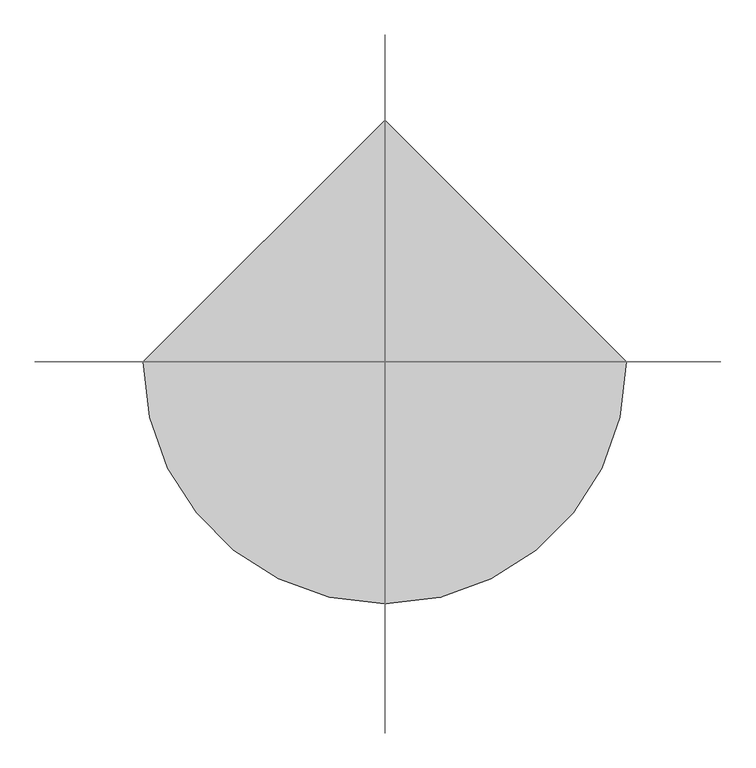
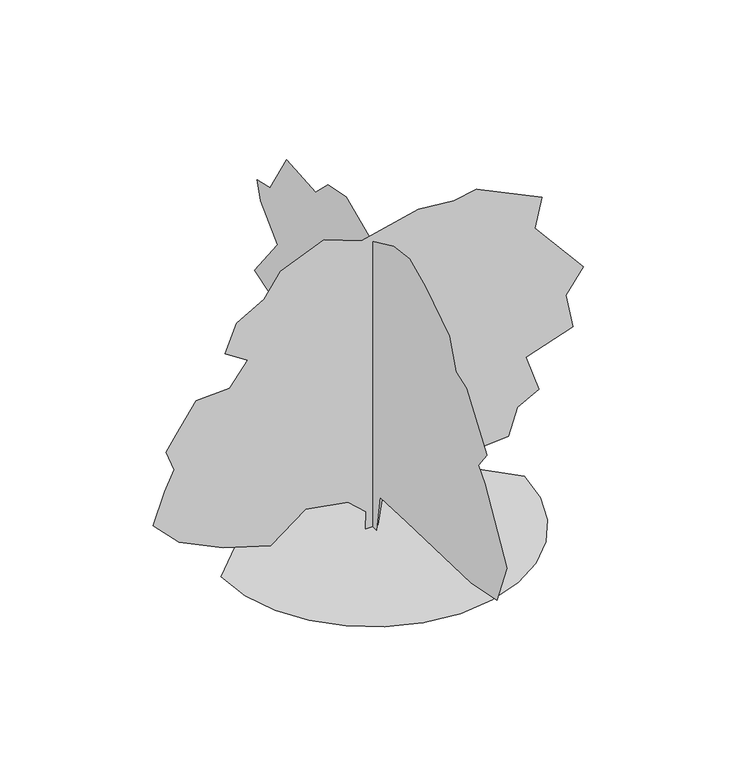
"""IFC4 building model written with IfcOpenShell, lengths in millimetres: proxy geometry, hibiscus syriacus 26076 : hibiscus syriacus 26076."""

import ifcopenshell
import ifcopenshell.guid

model = None  # the IFC model being written
_history = None  # IfcOwnerHistory: only IFC2X3 demands one
_inside = {}  # id of a spatial element -> (the spatial element, [elements in it])
_under = {}  # id of a project, library or spatial element -> (it, [spatial elements below it])
_declared = {}  # id of a project -> (the project, [libraries it declares])
_typed = {}  # id of a type object -> (the type object, [elements of that type])
_made_of = {}  # id of a material, layer set ... -> (it, [elements and type objects made of it])


def new_model(schema):
    """Start an empty IFC model of exactly this schema.

    Asked for "IFC4X3", IfcOpenShell would pick the latest addendum, in which some entities
    have other attributes; the version numbers below select the first issue.
    IFC2X3 requires an IfcOwnerHistory on every rooted entity: one is made here for all.
    """
    global model, _history
    if schema == "IFC4X3":
        model = ifcopenshell.file(schema_version=(4, 3, 0, 0))
    else:
        model = ifcopenshell.file(schema=schema)
    _inside.clear()
    _under.clear()
    _declared.clear()
    _typed.clear()
    _made_of.clear()
    _history = None
    if model.schema == "IFC2X3":
        org = make("IfcOrganization", Name="unknown")
        user = make(
            "IfcPersonAndOrganization",
            ThePerson=make("IfcPerson", FamilyName="unknown"),
            TheOrganization=org,
        )
        app = make(
            "IfcApplication",
            ApplicationDeveloper=org,
            Version="unknown",
            ApplicationFullName="unknown",
            ApplicationIdentifier="unknown",
        )
        _history = make(
            "IfcOwnerHistory",
            OwningUser=user,
            OwningApplication=app,
            ChangeAction="ADDED",
            CreationDate=0,
        )
    return model


def make(cls, **values):
    """One entity of the class cls with the attributes given. An attribute that is None is left unset."""
    return model.create_entity(
        cls, **{name: value for name, value in values.items() if value is not None}
    )


def rooted(cls, **values):
    """An entity with a GlobalId (a new one), such as an element, a storey or a relation."""
    return make(cls, GlobalId=ifcopenshell.guid.new(), OwnerHistory=_history, **values)


def si_unit(unit_type, name, prefix=None):
    """IfcSIUnit, for example si_unit("LENGTHUNIT", "METRE", prefix="MILLI")."""
    return make("IfcSIUnit", UnitType=unit_type, Prefix=prefix, Name=name)


def assignment(units):
    """IfcUnitAssignment: the units of a project."""
    return None if units is None else make("IfcUnitAssignment", Units=units)


def point(xyz):
    """IfcCartesianPoint."""
    return None if xyz is None else make("IfcCartesianPoint", Coordinates=xyz)


def direction(xyz):
    """IfcDirection."""
    return None if xyz is None else make("IfcDirection", DirectionRatios=xyz)


def frame(location, z_axis=None, x_axis=None):
    """IfcAxis2Placement3D, a coordinate frame: its origin and axes. An axis left out is left unset."""
    return make(
        "IfcAxis2Placement3D",
        Location=point(location),
        Axis=direction(z_axis),
        RefDirection=direction(x_axis),
    )


def origin():
    """The frame at (0, 0, 0) with its axes left unset."""
    return frame((0.0, 0.0, 0.0))


def place(relative_to, where):
    """IfcLocalPlacement: puts the frame where relative to a parent placement (None: the world)."""
    return make(
        "IfcLocalPlacement", PlacementRelTo=relative_to, RelativePlacement=where
    )


def context(
    kind, dimensions, precision=None, world=None, true_north=None, identifier=None
):
    """IfcGeometricRepresentationContext, for example the 3D "Model" context."""
    return make(
        "IfcGeometricRepresentationContext",
        ContextIdentifier=identifier,
        ContextType=kind,
        CoordinateSpaceDimension=dimensions,
        Precision=precision,
        WorldCoordinateSystem=world,
        TrueNorth=true_north,
    )


def project(units=None, contexts=None):
    """IfcProject with its units and contexts."""
    return rooted(
        "IfcProject",
        Name="project",
        RepresentationContexts=contexts,
        UnitsInContext=assignment(units),
    )


def spatial(cls, under=None, at=None, **own):
    """A site, building, storey or space (cls), placed at a placement, below another one or the project."""
    s = rooted(cls, ObjectPlacement=at, **own)
    if under is not None:
        _under.setdefault(under.id(), (under, []))[1].append(s)
    return s


def point_list(points):
    """IfcCartesianPointList2D or 3D."""
    cls = (
        "IfcCartesianPointList2D" if len(points[0]) == 2 else "IfcCartesianPointList3D"
    )
    return make(cls, CoordList=points)


def triangles(points, corners, closed=None, point_numbers=None):
    """IfcTriangulatedFaceSet: each triangle names its three corners, points numbered from 1."""
    return make(
        "IfcTriangulatedFaceSet",
        Coordinates=point_list(points),
        Closed=closed,
        CoordIndex=corners,
        PnIndex=point_numbers,
    )


def shape(context_of_items, identifier, shape_type, items):
    """IfcShapeRepresentation: the items that make up one representation, for example the "Body"."""
    return make(
        "IfcShapeRepresentation",
        ContextOfItems=context_of_items,
        RepresentationIdentifier=identifier,
        RepresentationType=shape_type,
        Items=items,
    )


def source(mapping_origin, context_of_items, identifier, shape_type, items):
    """IfcRepresentationMap: a shape defined once, which mapped items show again and again."""
    return make(
        "IfcRepresentationMap",
        MappingOrigin=mapping_origin,
        MappedRepresentation=shape(context_of_items, identifier, shape_type, items),
    )


def transform(
    local_origin,
    x_axis=None,
    y_axis=None,
    z_axis=None,
    scale=None,
    scale2=None,
    scale3=None,
    uniform=True,
):
    """IfcCartesianTransformationOperator3D, or its non-uniform kind. x_axis, y_axis, z_axis: its Axis1, 2, 3."""
    if uniform:
        return make(
            "IfcCartesianTransformationOperator3D",
            Axis1=direction(x_axis),
            Axis2=direction(y_axis),
            LocalOrigin=point(local_origin),
            Scale=scale,
            Axis3=direction(z_axis),
        )
    return make(
        "IfcCartesianTransformationOperator3DnonUniform",
        Axis1=direction(x_axis),
        Axis2=direction(y_axis),
        LocalOrigin=point(local_origin),
        Scale=scale,
        Axis3=direction(z_axis),
        Scale2=scale2,
        Scale3=scale3,
    )


def mapped(mapping_source, mapping_target):
    """IfcMappedItem: shows the shape of a source again, moved by a transform."""
    return make(
        "IfcMappedItem", MappingSource=mapping_source, MappingTarget=mapping_target
    )


def made_of(thing, what):
    """Note that an element or type object is made of a material, layer set ...; save() writes the relation."""
    if what is not None:
        _made_of.setdefault(what.id(), (what, []))[1].append(thing)
    return thing


def element(
    cls,
    number,
    at=None,
    inside=None,
    cuts=None,
    type_object=None,
    material=None,
    context=None,
    identifier="Body",
    shape_type=None,
    held_by="IfcProductDefinitionShape",
    body=None,
    shapes=None,
    **own,
):
    """One element of the class cls, such as IfcWall. Its Tag is "e" and its number.

    at: its placement. inside: the storey or other place that contains it. cuts: it is an
    opening in that element (IfcRelVoidsElement). A single representation is given by context,
    identifier, shape_type and body (its items); several are given by shapes. held_by: the class
    of the entity that holds the representations. save() writes the other relations.
    """
    e = rooted(cls, Tag="e%d" % number, ObjectPlacement=at, **own)
    if body is not None:
        shapes = [shape(context, identifier, shape_type, body)]
    if shapes is not None:
        e.Representation = make(held_by, Representations=shapes)
    if inside is not None:
        _inside.setdefault(inside.id(), (inside, []))[1].append(e)
    if cuts is not None:
        rooted(
            "IfcRelVoidsElement", RelatingBuildingElement=cuts, RelatedOpeningElement=e
        )
    if type_object is not None:
        _typed.setdefault(type_object.id(), (type_object, []))[1].append(e)
    return made_of(e, material)


def aggregate(whole, parts):
    """IfcRelAggregates: a whole, such as a stair, and the parts it consists of."""
    return rooted("IfcRelAggregates", RelatingObject=whole, RelatedObjects=parts)


def save(model, path):
    """Write the relations noted so far, then the file.

    IfcRelAggregates (storeys below a building ...), IfcRelContainedInSpatialStructure (elements
    in a storey), IfcRelDefinesByType, IfcRelAssociatesMaterial and IfcRelDeclares: one each for
    every whole, place, type object, material and project.
    """
    for whole, parts in _under.values():
        aggregate(whole, parts)
    for where, things in _inside.values():
        rooted(
            "IfcRelContainedInSpatialStructure",
            RelatedElements=things,
            RelatingStructure=where,
        )
    for kind, things in _typed.values():
        rooted("IfcRelDefinesByType", RelatedObjects=things, RelatingType=kind)
    for what, things in _made_of.values():
        rooted("IfcRelAssociatesMaterial", RelatedObjects=things, RelatingMaterial=what)
    for by, libraries in _declared.values():
        rooted("IfcRelDeclares", RelatingContext=by, RelatedDefinitions=libraries)
    model.write(path)


def entourage_edde2c96(model_context):
    return source(origin(), model_context, "Body", "Tessellation", [
        triangles([(-718.2296339, 0.0, 5.8e-05), (-699.2430748, -164.5709867, 5.8e-05), (-645.166361, -315.7023142, 5.8e-05), (-560.3301876, -449.0652858, 5.8e-05), (-449.0652858, -560.3301876, 5.8e-05), (-315.7023142, -645.166361, 5.8e-05), (-164.5707324, -699.2430748, 5.8e-05), (3.14e-05, -718.2296339, 5.8e-05), (164.5709867, -699.2430748, 5.8e-05), (315.7023142, -645.166361, 5.8e-05), (449.0652858, -560.3301876, 5.8e-05), (560.3301876, -449.0652858, 5.8e-05), (645.166361, -315.7023142, 5.8e-05), (699.2430748, -164.5707324, 5.8e-05), (718.2296339, 6.28e-05, 5.8e-05), (-9.42e-05, 718.2296339, 5.8e-05), (-34.4417068, 8.54e-05, 0.0004029), (-31.4201161, 7.54e-05, 85.3357887), (-116.0190539, 6.6e-05, 163.8917949), (-318.4505839, 6.17e-05, 200.1483391), (-484.6279043, 7.68e-05, 73.2501891), (-708.2093153, 6.85e-05, 142.7419322), (-916.6853256, 5.67e-05, 242.4475559), (-1040.5638834, 4.15e-05, 369.3446795), (-986.1773048, 2.35e-05, 520.4140194), (-940.856016, 1.24e-05, 614.076689), (-980.1346504, 1e-07, 716.8046482), (-931.7932697, -8.2e-06, 786.2967001), (-838.1305275, -2.47e-05, 925.2806585), (-677.9959705, -2.55e-05, 931.323313), (-593.398518, -3.84e-05, 1040.0939993), (-699.1465691, -4.67e-05, 1109.5859785), (-644.762534, -6.29e-05, 1245.5473743), (-514.8412491, -7.16e-05, 1318.0593727), (-436.2865236, -8.53e-05, 1432.8727135), (-230.8316043, -9.53e-05, 1517.4726368), (-52.5699789, -8.74e-05, 1451.0008221), (216.3332524, -9.5e-05, 1514.4501469), (385.5321362, -9.28e-05, 1496.3220383), (491.2801509, -9.53e-05, 1517.4726368), (802.4816133, -7.77e-05, 1369.4233887), (769.2456333, -6.04e-05, 1224.3967758), (998.8722422, -2.8e-05, 952.4739841), (914.2723188, -1.43e-05, 837.6606434), (947.5082262, 5.9e-06, 668.4632675), (726.946907, 1.49e-05, 592.9286339), (787.37614, 3.65e-05, 411.6459128), (684.6481808, 4.3e-05, 357.2593343), (642.3495272, 5.85e-05, 227.340611), (237.483106, 6.21e-05, 197.1267394), (140.7988277, 7.07e-05, 124.6136692), (53.1785627, 6.42e-05, 178.9984673), (25.9860297, 8.59e-05, 0.0), (-0.0007807, 31.0927106, 0.000457), (-0.0007807, 31.0927106, 100.9481805), (-0.0007869, 87.072138, 68.5389896), (-0.0007995, 193.1381747, 80.3241033), (-0.0008058, 269.7409118, 130.4109715), (-0.0008121, 346.3449205, 98.0017761), (-0.0008373, 520.1752622, 192.282958), (-0.0008373, 470.0888935, 354.3281542), (-0.0008562, 649.8120077, 383.7922351), (-0.0008688, 764.7167673, 489.857745), (-0.0008688, 747.0383406, 566.4617901), (-0.0008877, 891.4071447, 584.1376734), (-0.0008814, 850.1600258, 657.7952414), (-0.0009003, 970.9575943, 696.098572), (-0.0008877, 782.3951941, 937.693709), (-0.0009066, 920.8711893, 1073.2207563), (-0.0009066, 950.3327631, 1161.6103466), (-0.0009003, 841.3208124, 1188.1254433), (-0.000894, 705.7912216, 1409.0982925), (-0.0008688, 470.0888935, 1388.4733887), (-0.0008562, 366.9697881, 1488.6486694), (-0.0008436, 219.6545613, 1518.1102432), (-0.0008184, 4.575997, 1426.7767193), (-0.0007995, -172.2011714, 1509.2709572), (-0.0007869, -301.8364273, 1524.0030521), (-0.0007744, -431.473191, 1462.131102), (-0.0007492, -628.8747683, 1335.4407246), (-0.0007366, -684.8539822, 1191.0718477), (-0.0007303, -770.297168, 1161.6103466), (-0.0007051, -938.2346643, 925.9080185), (-0.0007114, -867.5235008, 834.5720238), (-0.0007051, -920.5562376, 772.700001), (-0.0006736, -1103.2258289, 460.3937004), (-0.0006736, -1020.7315184, 251.2085401), (-0.0006988, -811.5442869, 209.9606217), (-0.0007555, -275.3213124, 192.282958), (-0.0007744, -60.2420624, 183.443999), (-0.0007744, -30.7792736, 0.0004496)], [[15, 16, 1], [14, 15, 1], [14, 1, 2], [13, 14, 2], [13, 2, 3], [13, 3, 4], [12, 13, 4], [11, 12, 4], [11, 4, 5], [11, 5, 6], [11, 6, 7], [11, 7, 8], [11, 8, 9], [11, 9, 10], [53, 17, 18], [52, 53, 18], [52, 18, 19], [44, 45, 46], [46, 47, 48], [31, 32, 33], [40, 41, 42], [42, 43, 44], [31, 33, 34], [50, 51, 52], [48, 49, 50], [23, 24, 25], [46, 48, 50], [42, 44, 46], [39, 40, 42], [39, 42, 46], [39, 46, 50], [38, 39, 50], [37, 38, 50], [37, 50, 52], [37, 52, 19], [37, 19, 20], [36, 37, 20], [35, 36, 20], [34, 35, 20], [31, 34, 20], [30, 31, 20], [30, 20, 21], [30, 21, 22], [30, 22, 23], [30, 23, 25], [30, 25, 26], [29, 30, 26], [28, 29, 26], [28, 26, 27], [64, 65, 66], [66, 67, 68], [69, 70, 71], [91, 54, 55], [90, 91, 55], [68, 69, 71], [59, 60, 61], [58, 59, 61], [82, 83, 84], [71, 72, 73], [68, 71, 73], [64, 66, 68], [62, 63, 64], [86, 87, 88], [85, 86, 88], [85, 88, 89], [84, 85, 89], [82, 84, 89], [81, 82, 89], [81, 89, 90], [80, 81, 90], [79, 80, 90], [78, 79, 90], [77, 78, 90], [76, 77, 90], [75, 76, 90], [74, 75, 90], [73, 74, 90], [68, 73, 90], [64, 68, 90], [64, 90, 55], [64, 55, 56], [61, 62, 64], [61, 64, 56], [58, 61, 56], [58, 56, 57]], closed=False),
    ])


if __name__ == "__main__":
    model = new_model("IFC4")
    model_context = context("Model", 3, world=origin())
    ifc_project = project(units=[si_unit("LENGTHUNIT", "METRE", prefix="MILLI")], contexts=[model_context])
    site = spatial("IfcSite", under=ifc_project)
    building = spatial("IfcBuilding", under=site)
    placement = place(None, origin())
    entourage_shape = entourage_edde2c96(model_context)
    element("IfcBuildingElementProxy", 1, Name="hibiscus syriacus 26076 : hibiscus syriacus 26076", ObjectType="hibiscus syriacus 26076 : hibiscus syriacus 26076", at=placement, inside=building, context=model_context, shape_type="MappedRepresentation", body=[
        mapped(entourage_shape, transform((0.0, 0.0, 0.0), x_axis=(1.0, 0.0, 0.0), y_axis=(0.0, 1.0, 0.0), z_axis=(0.0, 0.0, 1.0))),
    ])
    save(model, "model.ifc")

# Revit data of these elements
# Type "hibiscus syriacus 26076 : hibiscus syriacus 26076"
#   built-in parameter 1005195 = "RPC-16-FVPE-AH00-2TUK-G000-ST1L-LVER-AU"
#   Height = 0
